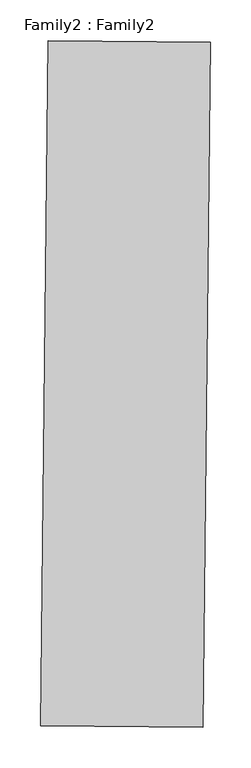
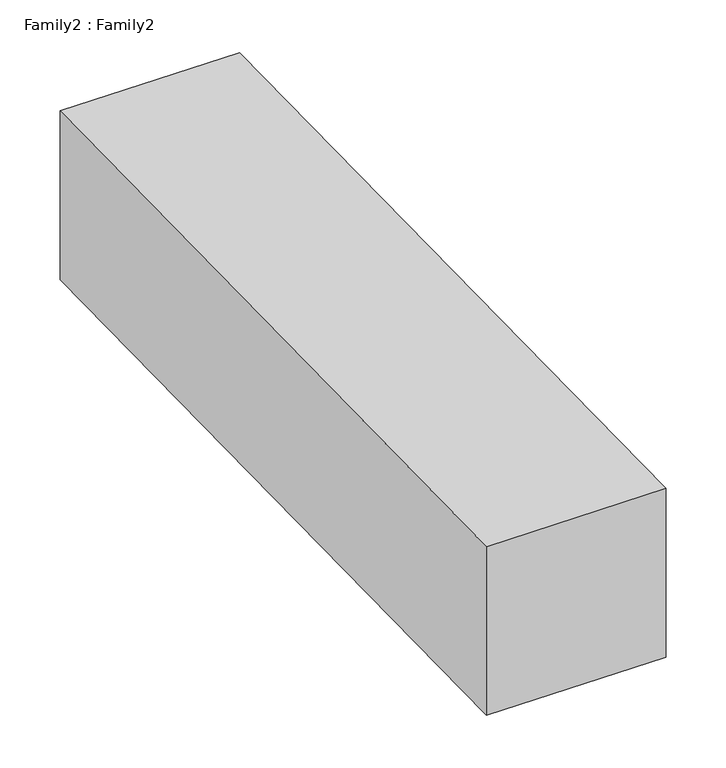
"""IFC4 building model written with IfcOpenShell, lengths in millimetres: proxy geometry, Family2 : Family2."""

import ifcopenshell
import ifcopenshell.guid

model = None  # the IFC model being written
_history = None  # IfcOwnerHistory: only IFC2X3 demands one
_inside = {}  # id of a spatial element -> (the spatial element, [elements in it])
_under = {}  # id of a project, library or spatial element -> (it, [spatial elements below it])
_declared = {}  # id of a project -> (the project, [libraries it declares])
_typed = {}  # id of a type object -> (the type object, [elements of that type])
_made_of = {}  # id of a material, layer set ... -> (it, [elements and type objects made of it])


def new_model(schema):
    """Start an empty IFC model of exactly this schema.

    Asked for "IFC4X3", IfcOpenShell would pick the latest addendum, in which some entities
    have other attributes; the version numbers below select the first issue.
    IFC2X3 requires an IfcOwnerHistory on every rooted entity: one is made here for all.
    """
    global model, _history
    if schema == "IFC4X3":
        model = ifcopenshell.file(schema_version=(4, 3, 0, 0))
    else:
        model = ifcopenshell.file(schema=schema)
    _inside.clear()
    _under.clear()
    _declared.clear()
    _typed.clear()
    _made_of.clear()
    _history = None
    if model.schema == "IFC2X3":
        org = make("IfcOrganization", Name="unknown")
        user = make(
            "IfcPersonAndOrganization",
            ThePerson=make("IfcPerson", FamilyName="unknown"),
            TheOrganization=org,
        )
        app = make(
            "IfcApplication",
            ApplicationDeveloper=org,
            Version="unknown",
            ApplicationFullName="unknown",
            ApplicationIdentifier="unknown",
        )
        _history = make(
            "IfcOwnerHistory",
            OwningUser=user,
            OwningApplication=app,
            ChangeAction="ADDED",
            CreationDate=0,
        )
    return model


def make(cls, **values):
    """One entity of the class cls with the attributes given. An attribute that is None is left unset."""
    return model.create_entity(
        cls, **{name: value for name, value in values.items() if value is not None}
    )


def rooted(cls, **values):
    """An entity with a GlobalId (a new one), such as an element, a storey or a relation."""
    return make(cls, GlobalId=ifcopenshell.guid.new(), OwnerHistory=_history, **values)


def si_unit(unit_type, name, prefix=None):
    """IfcSIUnit, for example si_unit("LENGTHUNIT", "METRE", prefix="MILLI")."""
    return make("IfcSIUnit", UnitType=unit_type, Prefix=prefix, Name=name)


def assignment(units):
    """IfcUnitAssignment: the units of a project."""
    return None if units is None else make("IfcUnitAssignment", Units=units)


def point(xyz):
    """IfcCartesianPoint."""
    return None if xyz is None else make("IfcCartesianPoint", Coordinates=xyz)


def direction(xyz):
    """IfcDirection."""
    return None if xyz is None else make("IfcDirection", DirectionRatios=xyz)


def frame(location, z_axis=None, x_axis=None):
    """IfcAxis2Placement3D, a coordinate frame: its origin and axes. An axis left out is left unset."""
    return make(
        "IfcAxis2Placement3D",
        Location=point(location),
        Axis=direction(z_axis),
        RefDirection=direction(x_axis),
    )


def origin():
    """The frame at (0, 0, 0) with its axes left unset."""
    return frame((0.0, 0.0, 0.0))


def place(relative_to, where):
    """IfcLocalPlacement: puts the frame where relative to a parent placement (None: the world)."""
    return make(
        "IfcLocalPlacement", PlacementRelTo=relative_to, RelativePlacement=where
    )


def context(
    kind, dimensions, precision=None, world=None, true_north=None, identifier=None
):
    """IfcGeometricRepresentationContext, for example the 3D "Model" context."""
    return make(
        "IfcGeometricRepresentationContext",
        ContextIdentifier=identifier,
        ContextType=kind,
        CoordinateSpaceDimension=dimensions,
        Precision=precision,
        WorldCoordinateSystem=world,
        TrueNorth=true_north,
    )


def project(units=None, contexts=None):
    """IfcProject with its units and contexts."""
    return rooted(
        "IfcProject",
        Name="project",
        RepresentationContexts=contexts,
        UnitsInContext=assignment(units),
    )


def spatial(cls, under=None, at=None, **own):
    """A site, building, storey or space (cls), placed at a placement, below another one or the project."""
    s = rooted(cls, ObjectPlacement=at, **own)
    if under is not None:
        _under.setdefault(under.id(), (under, []))[1].append(s)
    return s


def faces_of(points, faces, orient=None, outer=None):
    """IfcFace entities. A face is a list of loops; a loop is a list of indices into points, from 0.

    orient and outer hold one flag for each loop. By default every Orientation is true, the
    first loop of a face is its IfcFaceOuterBound and the others are IfcFaceBound.
    """
    made = []
    for i, loops in enumerate(faces):
        bounds = []
        for j, loop in enumerate(loops):
            is_outer = j == 0 if outer is None else outer[i][j]
            bounds.append(
                make(
                    "IfcFaceOuterBound" if is_outer else "IfcFaceBound",
                    Bound=make("IfcPolyLoop", Polygon=[points[k] for k in loop]),
                    Orientation=True if orient is None else orient[i][j],
                )
            )
        made.append(make("IfcFace", Bounds=bounds))
    return made


def faceted_brep(points, faces, orient=None, outer=None, voids=None):
    """IfcFacetedBrep: a solid bounded by flat faces; with voids (closed shells), ...WithVoids."""
    shared = [point(p) for p in points]
    hull = make("IfcClosedShell", CfsFaces=faces_of(shared, faces, orient, outer))
    if voids is None:
        return make("IfcFacetedBrep", Outer=hull)
    return make(
        "IfcFacetedBrepWithVoids",
        Outer=hull,
        Voids=[
            make(cls, CfsFaces=faces_of(shared, fs, o, b)) for cls, fs, o, b in voids
        ],
    )


def shape(context_of_items, identifier, shape_type, items):
    """IfcShapeRepresentation: the items that make up one representation, for example the "Body"."""
    return make(
        "IfcShapeRepresentation",
        ContextOfItems=context_of_items,
        RepresentationIdentifier=identifier,
        RepresentationType=shape_type,
        Items=items,
    )


def source(mapping_origin, context_of_items, identifier, shape_type, items):
    """IfcRepresentationMap: a shape defined once, which mapped items show again and again."""
    return make(
        "IfcRepresentationMap",
        MappingOrigin=mapping_origin,
        MappedRepresentation=shape(context_of_items, identifier, shape_type, items),
    )


def transform(
    local_origin,
    x_axis=None,
    y_axis=None,
    z_axis=None,
    scale=None,
    scale2=None,
    scale3=None,
    uniform=True,
):
    """IfcCartesianTransformationOperator3D, or its non-uniform kind. x_axis, y_axis, z_axis: its Axis1, 2, 3."""
    if uniform:
        return make(
            "IfcCartesianTransformationOperator3D",
            Axis1=direction(x_axis),
            Axis2=direction(y_axis),
            LocalOrigin=point(local_origin),
            Scale=scale,
            Axis3=direction(z_axis),
        )
    return make(
        "IfcCartesianTransformationOperator3DnonUniform",
        Axis1=direction(x_axis),
        Axis2=direction(y_axis),
        LocalOrigin=point(local_origin),
        Scale=scale,
        Axis3=direction(z_axis),
        Scale2=scale2,
        Scale3=scale3,
    )


def mapped(mapping_source, mapping_target):
    """IfcMappedItem: shows the shape of a source again, moved by a transform."""
    return make(
        "IfcMappedItem", MappingSource=mapping_source, MappingTarget=mapping_target
    )


def made_of(thing, what):
    """Note that an element or type object is made of a material, layer set ...; save() writes the relation."""
    if what is not None:
        _made_of.setdefault(what.id(), (what, []))[1].append(thing)
    return thing


def element(
    cls,
    number,
    at=None,
    inside=None,
    cuts=None,
    type_object=None,
    material=None,
    context=None,
    identifier="Body",
    shape_type=None,
    held_by="IfcProductDefinitionShape",
    body=None,
    shapes=None,
    **own,
):
    """One element of the class cls, such as IfcWall. Its Tag is "e" and its number.

    at: its placement. inside: the storey or other place that contains it. cuts: it is an
    opening in that element (IfcRelVoidsElement). A single representation is given by context,
    identifier, shape_type and body (its items); several are given by shapes. held_by: the class
    of the entity that holds the representations. save() writes the other relations.
    """
    e = rooted(cls, Tag="e%d" % number, ObjectPlacement=at, **own)
    if body is not None:
        shapes = [shape(context, identifier, shape_type, body)]
    if shapes is not None:
        e.Representation = make(held_by, Representations=shapes)
    if inside is not None:
        _inside.setdefault(inside.id(), (inside, []))[1].append(e)
    if cuts is not None:
        rooted(
            "IfcRelVoidsElement", RelatingBuildingElement=cuts, RelatedOpeningElement=e
        )
    if type_object is not None:
        _typed.setdefault(type_object.id(), (type_object, []))[1].append(e)
    return made_of(e, material)


def aggregate(whole, parts):
    """IfcRelAggregates: a whole, such as a stair, and the parts it consists of."""
    return rooted("IfcRelAggregates", RelatingObject=whole, RelatedObjects=parts)


def save(model, path):
    """Write the relations noted so far, then the file.

    IfcRelAggregates (storeys below a building ...), IfcRelContainedInSpatialStructure (elements
    in a storey), IfcRelDefinesByType, IfcRelAssociatesMaterial and IfcRelDeclares: one each for
    every whole, place, type object, material and project.
    """
    for whole, parts in _under.values():
        aggregate(whole, parts)
    for where, things in _inside.values():
        rooted(
            "IfcRelContainedInSpatialStructure",
            RelatedElements=things,
            RelatingStructure=where,
        )
    for kind, things in _typed.values():
        rooted("IfcRelDefinesByType", RelatedObjects=things, RelatingType=kind)
    for what, things in _made_of.values():
        rooted("IfcRelAssociatesMaterial", RelatedObjects=things, RelatingMaterial=what)
    for by, libraries in _declared.values():
        rooted("IfcRelDeclares", RelatingContext=by, RelatedDefinitions=libraries)
    model.write(path)


def family2_family2_f9c1c3c1(model_context):
    return source(origin(), model_context, "Body", "Brep", [
        faceted_brep([(-3948.1947636, -6495.5551337, 1.0945136), (-3948.1947636, -6495.5551337, 201.0945136), (-3938.6480309, -5652.0449889, 202.060409), (-3938.6480309, -5652.0449889, 2.060409), (-3748.2035736, -6497.4323464, 201.0945136), (-3738.6568409, -5653.9222016, 202.060409), (-3748.2035736, -6497.4323464, 1.0945136), (-3738.6568409, -5653.9222016, 2.060409)], [[[0, 1, 2, 3]], [[1, 4, 5, 2]], [[4, 6, 7, 5]], [[6, 0, 3, 7]], [[3, 2, 5, 7]], [[0, 6, 4, 1]]]),
    ])


if __name__ == "__main__":
    model = new_model("IFC4")
    model_context = context("Model", 3, world=origin())
    ifc_project = project(units=[si_unit("LENGTHUNIT", "METRE", prefix="MILLI")], contexts=[model_context])
    site = spatial("IfcSite", under=ifc_project)
    building = spatial("IfcBuilding", under=site)
    placement = place(None, origin())
    family2_family2_shape = family2_family2_f9c1c3c1(model_context)
    element("IfcBuildingElementProxy", 1, Name="Family2 : Family2", ObjectType="Family2 : Family2", at=placement, inside=building, context=model_context, shape_type="MappedRepresentation", body=[
        mapped(family2_family2_shape, transform((0.0, 0.0, 0.0), x_axis=(1.0, 0.0, 0.0), y_axis=(0.0, 1.0, 0.0), z_axis=(0.0, 0.0, 1.0))),
    ])
    save(model, "model.ifc")

# Revit data of these elements
# Type "Family2 : Family2"
#   Default Elevation = 0
